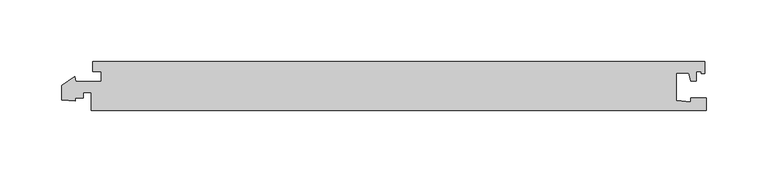
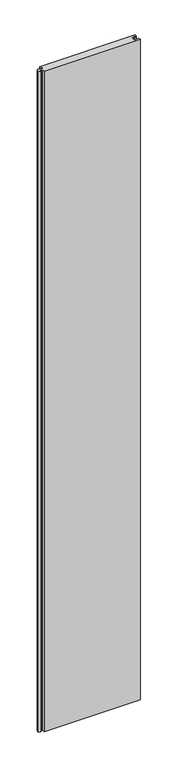
"""IFC4 building model written with IfcOpenShell, lengths in millimetres: proxy geometry, Generic Models 5:Generic Models 5:321804:Generic Models 5:321804 : Generic Models 5:Generic Models 5:321804:7 : Generic Models 5:Generic Models 5:321804:Generic Models 5:321804 : Generic Models 5:Generic Models 5:321804:300761."""

from ifc_helpers import new_model, si_unit, frame, origin, place, context, project, spatial, polyline, outline, extrude, source, transform, mapped, element, save


def generic_models_cda98ae3(model_context):
    return source(origin(), model_context, "Body", "SweptSolid", [
        extrude(outline(polyline([(592720.2261126, -579052.1037319), (592709.8677824, -579052.1037319), (592709.8677824, -579074.5995222), (592721.8677824, -579075.6493861), (592721.8677824, -579072.4037319), (592734.6177824, -579072.4037319), (592734.6177824, -579082.6037319), (592234.6177824, -579082.6037319), (592234.6177824, -579068.1037319), (592227.9927824, -579068.1037319), (592227.9927824, -579072.4037319), (592221.3677824, -579072.4037319), (592221.3677824, -579075.1037319), (592210.3677824, -579074.1413566), (592210.3677824, -579062.2832156), (592221.0492843, -579055.1758504), (592222.101757, -579059.1037319), (592242.8177824, -579059.1037319), (592242.8177824, -579051.1037319), (592235.8677824, -579051.1037319), (592235.8677824, -579042.6037319), (592733.3677824, -579042.6037319), (592733.3677824, -579052.6037319), (592730.3677824, -579052.6037319), (592730.3677824, -579051.1037319), (592726.4177824, -579051.1037319), (592726.4177824, -579058.6037319), (592721.9677824, -579058.6037319), (592720.2261126, -579052.1037319)])), frame((0.0, 0.0, 30.0324973), z_axis=(0.0, 0.0, 1.0), x_axis=(1.0, 0.0, 0.0)), (0.0, 0.0, 1.0), 3634.8310765),
    ])


if __name__ == "__main__":
    model = new_model("IFC4")
    model_context = context("Model", 3, world=origin())
    ifc_project = project(units=[si_unit("LENGTHUNIT", "METRE", prefix="MILLI")], contexts=[model_context])
    site = spatial("IfcSite", under=ifc_project)
    building = spatial("IfcBuilding", under=site)
    placement = place(None, origin())
    generic_models_shape = generic_models_cda98ae3(model_context)
    element("IfcBuildingElementProxy", 1, Name="Generic Models 5:Generic Models 5:321804:Generic Models 5:321804 : Generic Models 5:Generic Models 5:321804:7 : Generic Models 5:Generic Models 5:321804:Generic Models 5:321804 : Generic Models 5:Generic Models 5:321804:300761", ObjectType="Generic Models 5:Generic Models 5:321804:Generic Models 5:321804 : Generic Models 5:Generic Models 5:321804:7 : Generic Models 5:Generic Models 5:321804:Generic Models 5:321804 : Generic Models 5:Generic Models 5:321804:300761", at=placement, inside=building, context=model_context, shape_type="MappedRepresentation", body=[
        mapped(generic_models_shape, transform((0.0, 0.0, 0.0), x_axis=(1.0, 0.0, 0.0), y_axis=(0.0, 1.0, 0.0), z_axis=(0.0, 0.0, 1.0))),
    ])
    save(model, "model.ifc")

# Revit data of these elements
# Type "Generic Models 5:Generic Models 5:321804:Generic Models 5:321804 : Generic Models 5:Generic Models 5:321804:7 : Generic Models 5:Generic Models 5:321804:Generic Models 5:321804 : Generic Models 5:Generic Models 5:321804:300761"
#   NameOverride = "Generic Models 5:Generic Models 5:321804:Generic Models 5:321804 : Generic Models 5:Generic Models 5:321804:300761"
#   ObjectTypeOverride = "Generic Models 5:321804 : Generic Models 5:Generic Models 5:321804"
#   Reference = "Generic Models 5"
#   Tag = "300761"
# Element 1 (IfcBuildingElementProxy, "Generic Models 5:Generic Models 5:321804:Generic Models 5:321804 : Generic Models 5:Generic Models 5:321804:7 : Generic Models 5:Generic Models 5:321804:Generic Models 5:321804 : Generic Models 5:Generic Models 5:321804:300761")
#   Materials on its faces: "POLYCARBONATE PANEL - ARCOPLUS 547"
# Materials
#   "POLYCARBONATE PANEL - ARCOPLUS 547": class "Unassigned", colour RGB 202 225 249, transparency 0.45, Cost = 0
